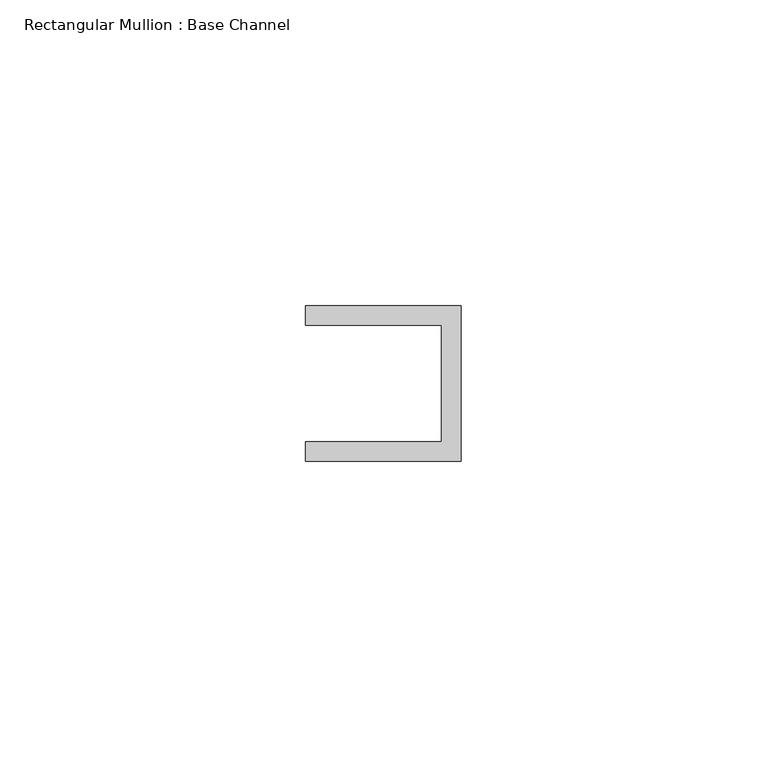
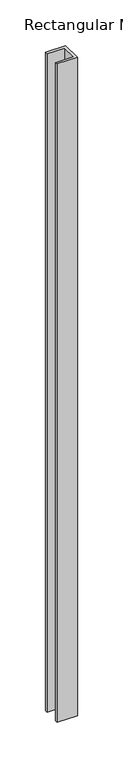
"""IFC4 building model written with IfcOpenShell, lengths in millimetres: member geometry, Rectangular Mullion : Base Channel."""

from ifc_helpers import new_model, si_unit, frame, origin, place, context, project, spatial, polyline, outline, extrude, source, transform, mapped, element, save


def rectangular_mullion_base_channel_16ec950e(model_context):
    return source(origin(), model_context, "Body", "SweptSolid", [
        extrude(outline(polyline([(0.0, -12.7), (-25.4, -12.7), (-25.4, -9.525), (-3.175, -9.525), (-3.175, 9.525), (-25.4, 9.525), (-25.4, 12.7), (0.0, 12.7), (0.0, -12.7)])), frame((0.0, 0.0, -877.8332392), z_axis=(0.0, 0.0, 1.0), x_axis=(1.0, 0.0, 0.0)), (0.0, 0.0, 1.0), 877.8332392),
    ])


if __name__ == "__main__":
    model = new_model("IFC4")
    model_context = context("Model", 3, world=origin())
    ifc_project = project(units=[si_unit("LENGTHUNIT", "METRE", prefix="MILLI")], contexts=[model_context])
    site = spatial("IfcSite", under=ifc_project)
    building = spatial("IfcBuilding", under=site)
    placement = place(None, origin())
    rectangular_mullion_base_channel_shape = rectangular_mullion_base_channel_16ec950e(model_context)
    element("IfcMember", 1, ObjectType="Rectangular Mullion : Base Channel", at=placement, inside=building, context=model_context, shape_type="MappedRepresentation", body=[
        mapped(rectangular_mullion_base_channel_shape, transform((0.0, 0.0, 0.0), x_axis=(1.0, 0.0, 0.0), y_axis=(0.0, 1.0, 0.0), z_axis=(0.0, 0.0, 1.0))),
    ])
    save(model, "model.ifc")

# Revit data of these elements
# Type "Rectangular Mullion : Base Channel"
#   built-in parameter 1007322 = 0.0833333 (stored number, unit not read)
#   built-in parameter 1007321 = 0.0416667 (stored number, unit not read)
#   built-in parameter 1007320 = -0.03125 (stored number, unit not read)
# Element 1 (IfcMember, "Rectangular Mullion : Base Channel")
#   Materials on its faces: "ALUM"
# Materials
#   "ALUM": class "Generic", colour RGB 157 157 157, transparency 0, Cost = 0
